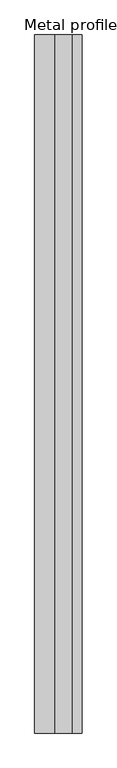
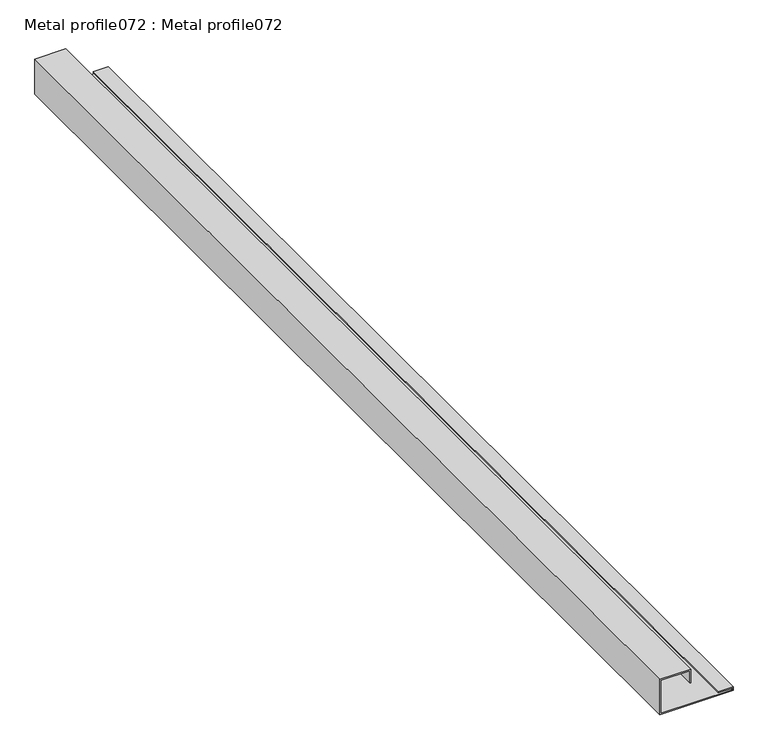
"""IFC4 building model written with IfcOpenShell, lengths in millimetres: proxy geometry, Metal profile072 : Metal profile072."""

from ifc_helpers import new_model, si_unit, frame, origin, place, context, project, spatial, polyline, outline, extrude, source, transform, mapped, element, save


def metal_profile072_metal_profile072_a42efd89(model_context):
    return source(origin(), model_context, "Body", "SweptSolid", [
        extrude(outline(polyline([(43450.8984375, -6380.8935547), (43450.8984375, -6355.1303711), (43448.03125, -6355.1303711), (43448.03125, -6486.7294922), (43512.8046875, -6486.7294922), (43512.8046875, -6433.3842773), (43488.7109375, -6433.3842773), (43488.7109375, -6431.3842773), (43514.8046875, -6431.3842773), (43514.8046875, -6488.7294922), (43446.03125, -6488.7294922), (43446.03125, -6353.1303711), (43452.8984375, -6353.1303711), (43452.8984375, -6380.8935547), (43450.8984375, -6380.8935547)])), frame((0.0, 7982.1531721, 0.0), z_axis=(0.0, 1.0, 0.0), x_axis=(0.0, 0.0, 1.0)), (0.0, 0.0, 1.0), 2000.0),
    ])


if __name__ == "__main__":
    model = new_model("IFC4")
    model_context = context("Model", 3, world=origin())
    ifc_project = project(units=[si_unit("LENGTHUNIT", "METRE", prefix="MILLI")], contexts=[model_context])
    site = spatial("IfcSite", under=ifc_project)
    building = spatial("IfcBuilding", under=site)
    placement = place(None, origin())
    metal_profile072_metal_profile072_shape = metal_profile072_metal_profile072_a42efd89(model_context)
    element("IfcBuildingElementProxy", 1, Name="Metal profile072 : Metal profile072", ObjectType="Metal profile072 : Metal profile072", at=placement, inside=building, context=model_context, shape_type="MappedRepresentation", body=[
        mapped(metal_profile072_metal_profile072_shape, transform((0.0, 0.0, 0.0), x_axis=(1.0, 0.0, 0.0), y_axis=(0.0, 1.0, 0.0), z_axis=(0.0, 0.0, 1.0))),
    ])
    save(model, "model.ifc")

# Revit data of these elements
# Type "Metal profile072 : Metal profile072"
#   NameOverride = "Metal profile072"
# Element 1 (IfcBuildingElementProxy, "Metal profile072 : Metal profile072")
#   Materials on its faces: "RECEIVER TRIM"
# Materials
#   "RECEIVER TRIM": class "Unassigned", colour RGB 255 250 0, transparency 0
